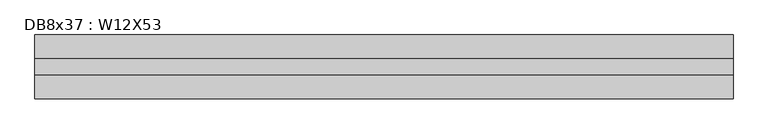
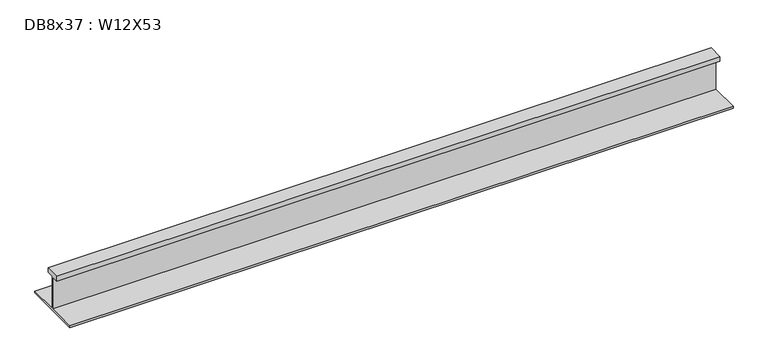
"""IFC4 building model written with IfcOpenShell, lengths in millimetres: beam geometry, DB8x37 : W12X53."""

from ifc_helpers import new_model, si_unit, frame, origin, place, context, project, spatial, polyline, outline, extrude, source, transform, mapped, element, save


def db8x37_w12x53_14e4f451(model_context):
    return source(origin(), model_context, "Body", "SweptSolid", [
        extrude(outline(polyline([(38.1, 145.415), (38.1, 120.015), (2.921, 120.015), (2.921, -48.4505), (152.4, -48.4505), (152.4, -58.1025), (-152.4, -58.1025), (-152.4, -48.4505), (-2.921, -48.4505), (-2.921, 120.015), (-38.1, 120.015), (-38.1, 145.415), (38.1, 145.415)])), frame((-1663.573, 0.0, 0.0), z_axis=(1.0, 0.0, 0.0), x_axis=(0.0, 1.0, 0.0)), (0.0, 0.0, 1.0), 3327.146),
    ])


if __name__ == "__main__":
    model = new_model("IFC4")
    model_context = context("Model", 3, world=origin())
    ifc_project = project(units=[si_unit("LENGTHUNIT", "METRE", prefix="MILLI")], contexts=[model_context])
    site = spatial("IfcSite", under=ifc_project)
    building = spatial("IfcBuilding", under=site)
    placement = place(None, origin())
    db8x37_w12x53_shape = db8x37_w12x53_14e4f451(model_context)
    element("IfcBeam", 1, ObjectType="DB8x37 : W12X53", at=placement, inside=building, context=model_context, shape_type="MappedRepresentation", body=[
        mapped(db8x37_w12x53_shape, transform((0.0, 0.0, 0.0), x_axis=(1.0, 0.0, 0.0), y_axis=(0.0, 1.0, 0.0), z_axis=(0.0, 0.0, 1.0))),
    ])
    save(model, "model.ifc")

# Revit data of these elements
# Type "DB8x37 : W12X53"
#   Assembly Code = "B10"
#   W = 53
#   Length [instance default] = 5' - 0"
#   bf = 0' - 10"
#   d = 1' - 0.1"
#   k = 0' - 1 3/8"
#   k2 = 0' - 0.8"
#   tf = 0' - 0.575"
#   tw = 0' - 0.345"
#   A = 0.108333 SF
#   Structural Material [instance default] = Steel ASTM A992
# Element 1 (IfcBeam, "DB8x37 : W12X53")
#   Materials on its faces: "Steel ASTM A992"
# Materials
#   "Steel ASTM A992": class "Metal", colour RGB 199 199 199, transparency 0, Description = "Structural steel 50ksi", Cost = 0
